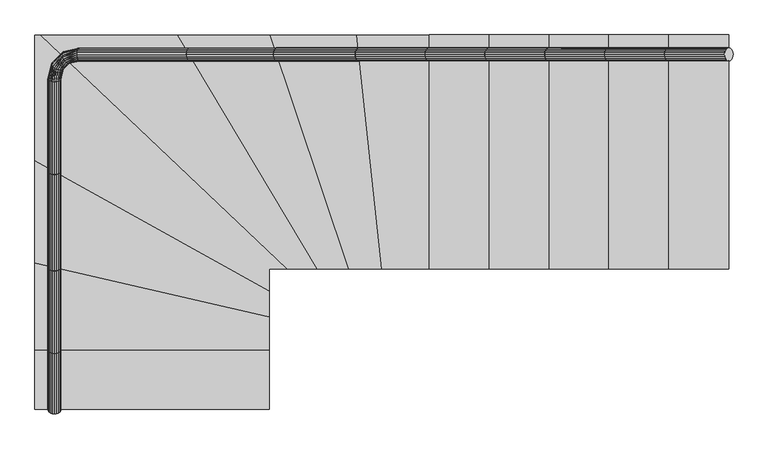
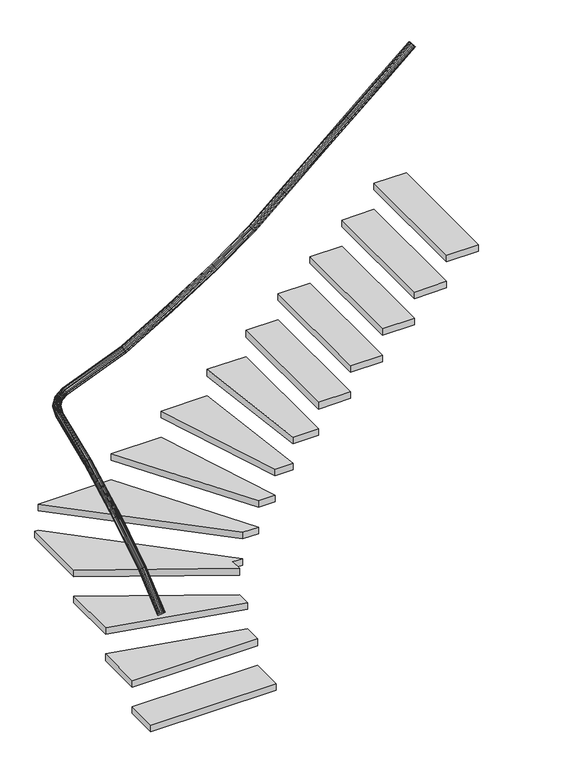
"""IFC4 building model written with IfcOpenShell, lengths in millimetres: stair geometry, 0_3d."""

from ifc_helpers import new_model, si_unit, frame, origin, origin_with_axes, place, context, project, spatial, polyline, outline, extrude, faceted_brep, source, transform, mapped, element, save


def stair_7a128c32(model_context):
    return source(origin(), model_context, "Body", "SolidModel", [
        faceted_brep([(51.2235871, 11.6788974, 875.6088541), (50.0, 16.9018591, 869.5592366), (51.2235871, 22.1248208, 863.5096191), (54.7745751, 26.8365226, 858.0521803), (60.3053687, 30.5757504, 853.7211323), (67.2745751, 32.9764824, 850.9404284), (75.0, 33.8037182, 849.9822631), (82.7254249, 32.9764824, 850.9404284), (89.6946313, 30.5757504, 853.7211323), (95.2254249, 26.8365226, 858.0521803), (98.7764129, 22.1248208, 863.5096191), (100.0, 16.9018591, 869.5592366), (98.7764129, 11.6788974, 875.6088541), (95.2254249, 6.9671956, 881.0662929), (89.6946313, 3.2279679, 885.3973409), (82.7254249, 0.8272359, 888.1780448), (75.0, 0.0, 889.1362101), (67.2745751, 0.8272359, 888.1780448), (60.3053687, 3.2279679, 885.3973409), (54.7745751, 6.9671956, 881.0662929), (51.2235871, 251.6675536, 1061.6862641), (50.0, 246.9018591, 1068.1306652), (51.2235871, 242.1361647, 1074.5750662), (54.7745751, 237.8369696, 1080.3886444), (60.3053687, 234.4251091, 1085.0023262), (67.2745751, 232.2345598, 1087.9644922), (75.0, 231.4797479, 1088.985185), (82.7254249, 232.2345598, 1087.9644922), (89.6946313, 234.4251091, 1085.0023262), (95.2254249, 237.8369696, 1080.3886444), (98.7764129, 242.1361647, 1074.5750662), (100.0, 246.9018591, 1068.1306652), (98.7764129, 251.6675536, 1061.6862641), (95.2254249, 255.9667486, 1055.872686), (89.6946313, 259.3786091, 1051.2590042), (82.7254249, 261.5691584, 1048.2968382), (75.0, 262.3239703, 1047.2761453), (67.2745751, 261.5691584, 1048.2968382), (60.3053687, 259.3786091, 1051.2590042), (54.7745751, 255.9667486, 1055.872686)], [[[0, 1, 2, 3, 4, 5, 6, 7, 8, 9, 10, 11, 12, 13, 14, 15, 16, 17, 18, 19]], [[20, 21, 22, 23, 24, 25, 26, 27, 28, 29, 30, 31, 32, 33, 34, 35, 36, 37, 38, 39]], [[21, 1, 0, 22]], [[22, 0, 19, 23]], [[23, 19, 18, 24]], [[24, 18, 17, 25]], [[25, 17, 16, 26]], [[26, 16, 15, 27]], [[27, 15, 14, 28]], [[28, 14, 13, 29]], [[29, 13, 12, 30]], [[30, 12, 11, 31]], [[31, 11, 10, 32]], [[32, 10, 9, 33]], [[33, 9, 8, 34]], [[34, 8, 7, 35]], [[35, 7, 6, 36]], [[36, 6, 5, 37]], [[37, 5, 4, 38]], [[38, 4, 3, 39]], [[39, 3, 2, 20]], [[20, 2, 1, 21]]]),
        extrude(outline(polyline([(900.0, 373.9346688), (0.0, 579.8690495), (0.0, 973.1970565), (900.0, 473.824936), (900.0, 373.9346688)])), frame((0.0, 0.0, 397.1428571), z_axis=(0.0, 0.0, 1.0), x_axis=(1.0, 0.0, 0.0)), (0.0, 0.0, 1.0), 50.0),
        extrude(outline(polyline([(1.2235871, -7.9923214), (0.0, 0.0), (1.2235871, 7.9923214), (4.7745751, 15.2022986), (10.3053687, 20.924169), (17.2745751, 24.5978359), (25.0, 25.8636953), (32.7254248, 24.5978359), (39.6946313, 20.924169), (45.2254248, 15.2022986), (48.7764129, 7.9923214), (50.0, 0.0), (48.7764129, -7.9923214), (45.2254248, -15.2022987), (39.6946313, -20.9241691), (32.7254248, -24.597836), (25.0, -25.8636953), (17.2745751, -24.597836), (10.3053687, -20.9241691), (4.7745751, -15.2022987), (1.2235871, -7.9923214)])), frame((1744.6018366, 1406.9018591, 2656.7020937), z_axis=(0.7569287102857354, 0.0, 0.6534974579485168), x_axis=(0.0, -1.0, 0.0)), (0.0, 0.0, 1.0), 303.8595272),
        faceted_brep([(1509.6138519, 1405.678272, 2464.383151), (1514.6018366, 1406.9018591, 2458.1306652), (1519.5898213, 1405.678272, 2451.8781793), (1524.0895473, 1402.127284, 2446.2377304), (1527.6605501, 1396.5964904, 2441.7614447), (1529.9532751, 1389.627284, 2438.8874925), (1530.7432942, 1381.9018591, 2437.897196), (1529.9532751, 1374.1764343, 2438.8874925), (1527.6605501, 1367.2072278, 2441.7614447), (1524.0895473, 1361.6764343, 2446.2377304), (1519.5898213, 1358.1254462, 2451.8781793), (1514.6018366, 1356.9018591, 2458.1306652), (1509.6138519, 1358.1254462, 2464.383151), (1505.1141259, 1361.6764343, 2470.0236), (1501.5431231, 1367.2072278, 2474.4998856), (1499.2503981, 1374.1764343, 2477.3738379), (1498.460379, 1381.9018591, 2478.3641344), (1499.2503981, 1389.627284, 2477.3738379), (1501.5431231, 1396.5964904, 2474.4998856), (1505.1141259, 1402.127284, 2470.0236), (1749.8247983, 1405.678272, 2650.6524762), (1744.6018366, 1406.9018591, 2656.7020937), (1739.3788749, 1405.678272, 2662.7517113), (1734.6671731, 1402.127284, 2668.2091501), (1730.9279453, 1396.5964904, 2672.540198), (1728.5272134, 1389.627284, 2675.320902), (1727.6999775, 1381.9018591, 2676.2790673), (1728.5272134, 1374.1764343, 2675.320902), (1730.9279453, 1367.2072278, 2672.540198), (1734.6671731, 1361.6764343, 2668.2091501), (1739.3788749, 1358.1254462, 2662.7517113), (1744.6018366, 1356.9018591, 2656.7020937), (1749.8247983, 1358.1254462, 2650.6524762), (1754.5365001, 1361.6764343, 2645.1950374), (1758.2757279, 1367.2072278, 2640.8639895), (1760.6764598, 1374.1764343, 2638.0832855), (1761.5036957, 1381.9018591, 2637.1251202), (1760.6764598, 1389.627284, 2638.0832855), (1758.2757279, 1396.5964904, 2640.8639895), (1754.5365001, 1402.127284, 2645.1950374)], [[[0, 1, 2, 3, 4, 5, 6, 7, 8, 9, 10, 11, 12, 13, 14, 15, 16, 17, 18, 19]], [[20, 21, 22, 23, 24, 25, 26, 27, 28, 29, 30, 31, 32, 33, 34, 35, 36, 37, 38, 39]], [[21, 1, 0, 22]], [[22, 0, 19, 23]], [[23, 19, 18, 24]], [[24, 18, 17, 25]], [[25, 17, 16, 26]], [[26, 16, 15, 27]], [[27, 15, 14, 28]], [[28, 14, 13, 29]], [[29, 13, 12, 30]], [[30, 12, 11, 31]], [[31, 11, 10, 32]], [[32, 10, 9, 33]], [[33, 9, 8, 34]], [[34, 8, 7, 35]], [[35, 7, 6, 36]], [[36, 6, 5, 37]], [[37, 5, 4, 38]], [[38, 4, 3, 39]], [[39, 3, 2, 20]], [[20, 2, 1, 21]]]),
        faceted_brep([(51.2235871, 242.1361647, 1074.5750662), (50.0, 246.9018591, 1068.1306652), (51.2235871, 251.6675536, 1061.6862641), (54.7745751, 255.9667486, 1055.872686), (60.3053687, 259.3786091, 1051.2590042), (67.2745751, 261.5691584, 1048.2968382), (75.0, 262.3239703, 1047.2761453), (82.7254249, 261.5691584, 1048.2968382), (89.6946313, 259.3786091, 1051.2590042), (95.2254249, 255.9667486, 1055.872686), (98.7764129, 251.6675536, 1061.6862641), (100.0, 246.9018591, 1068.1306652), (98.7764129, 242.1361647, 1074.5750662), (95.2254249, 237.8369696, 1080.3886444), (89.6946313, 234.4251091, 1085.0023262), (82.7254249, 232.2345598, 1087.9644922), (75.0, 231.4797479, 1088.985185), (67.2745751, 232.2345598, 1087.9644922), (60.3053687, 234.4251091, 1085.0023262), (54.7745751, 237.8369696, 1080.3886444), (51.2235871, 566.7337566, 1259.7925307), (50.0, 562.7078511, 1266.7020937), (51.2235871, 558.6819455, 1273.6116568), (54.7745751, 555.0501237, 1279.8448636), (60.3053687, 552.1678935, 1284.7915646), (67.2745751, 550.3173878, 1287.9675421), (75.0, 549.679747, 1289.0619094), (82.7254249, 550.3173878, 1287.9675421), (89.6946313, 552.1678935, 1284.7915646), (95.2254249, 555.0501237, 1279.8448636), (98.7764129, 558.6819455, 1273.6116568), (100.0, 562.7078511, 1266.7020937), (98.7764129, 566.7337566, 1259.7925307), (95.2254249, 570.3655785, 1253.5593239), (89.6946313, 573.2478087, 1248.6126229), (82.7254249, 575.0983143, 1245.4366454), (75.0, 575.7359551, 1244.3422781), (67.2745751, 575.0983143, 1245.4366454), (60.3053687, 573.2478087, 1248.6126229), (54.7745751, 570.3655785, 1253.5593239)], [[[0, 1, 2, 3, 4, 5, 6, 7, 8, 9, 10, 11, 12, 13, 14, 15, 16, 17, 18, 19]], [[20, 21, 22, 23, 24, 25, 26, 27, 28, 29, 30, 31, 32, 33, 34, 35, 36, 37, 38, 39]], [[21, 1, 0, 22]], [[22, 0, 19, 23]], [[23, 19, 18, 24]], [[24, 18, 17, 25]], [[25, 17, 16, 26]], [[26, 16, 15, 27]], [[27, 15, 14, 28]], [[28, 14, 13, 29]], [[29, 13, 12, 30]], [[30, 12, 11, 31]], [[31, 11, 10, 32]], [[32, 10, 9, 33]], [[33, 9, 8, 34]], [[34, 8, 7, 35]], [[35, 7, 6, 36]], [[36, 6, 5, 37]], [[37, 5, 4, 38]], [[38, 4, 3, 39]], [[39, 3, 2, 20]], [[20, 2, 1, 21]]]),
        extrude(outline(polyline([(1.2235871, -7.9923214), (0.0, 0.0), (1.2235871, 7.9923214), (4.7745751, 15.2022986), (10.3053687, 20.9241691), (17.2745751, 24.597836), (25.0, 25.8636953), (32.7254248, 24.597836), (39.6946313, 20.9241691), (45.2254248, 15.2022986), (48.7764129, 7.9923214), (50.0, 0.0), (48.7764129, -7.9923214), (45.2254248, -15.2022986), (39.6946313, -20.924169), (32.7254248, -24.5978359), (25.0, -25.8636953), (17.2745751, -24.5978359), (10.3053687, -20.924169), (4.7745751, -15.2022986), (1.2235871, -7.9923214)])), frame((2434.6018366, 1406.9018591, 3252.4163795), z_axis=(0.7569287102857536, 0.0, 0.6534974579484957), x_axis=(0.0, -1.0, 0.0)), (0.0, 0.0, 1.0), 303.8595272),
        faceted_brep([(925.538539, 1405.678272, 2067.8109967), (929.7020117, 1406.9018591, 2060.987808), (933.8654844, 1405.678272, 2054.1646194), (937.6214074, 1402.127284, 2048.009332), (940.6021247, 1396.5964904, 2043.1244683), (942.515863, 1389.627284, 2039.9881928), (943.1752923, 1381.9018591, 2038.9075058), (942.515863, 1374.1764343, 2039.9881928), (940.6021247, 1367.2072278, 2043.1244683), (937.6214074, 1361.6764343, 2048.009332), (933.8654844, 1358.1254462, 2054.1646194), (929.7020117, 1356.9018591, 2060.987808), (925.538539, 1358.1254462, 2067.8109967), (921.782616, 1361.6764343, 2073.966284), (918.8018987, 1367.2072278, 2078.8511477), (916.8881603, 1374.1764343, 2081.9874233), (916.228731, 1381.9018591, 2083.0681102), (916.8881603, 1389.627284, 2081.9874233), (918.8018987, 1396.5964904, 2078.8511477), (921.782616, 1402.127284, 2073.966284), (1249.3489942, 1405.678272, 2252.9513864), (1244.8437697, 1406.9018591, 2259.5592366), (1240.3385453, 1405.678272, 2266.1670868), (1236.2743236, 1402.127284, 2272.1281145), (1233.048939, 1396.5964904, 2276.858813), (1230.9781146, 1389.627284, 2279.8961083), (1230.2645572, 1381.9018591, 2280.942689), (1230.9781146, 1374.1764343, 2279.8961083), (1233.048939, 1367.2072278, 2276.858813), (1236.2743236, 1361.6764343, 2272.1281145), (1240.3385453, 1358.1254462, 2266.1670868), (1244.8437697, 1356.9018591, 2259.5592366), (1249.3489942, 1358.1254462, 2252.9513864), (1253.4132159, 1361.6764343, 2246.9903587), (1256.6386004, 1367.2072278, 2242.2596602), (1258.7094248, 1374.1764343, 2239.2223649), (1259.4229823, 1381.9018591, 2238.1757842), (1258.7094248, 1389.627284, 2239.2223649), (1256.6386004, 1396.5964904, 2242.2596602), (1253.4132159, 1402.127284, 2246.9903587)], [[[0, 1, 2, 3, 4, 5, 6, 7, 8, 9, 10, 11, 12, 13, 14, 15, 16, 17, 18, 19]], [[20, 21, 22, 23, 24, 25, 26, 27, 28, 29, 30, 31, 32, 33, 34, 35, 36, 37, 38, 39]], [[21, 1, 0, 22]], [[22, 0, 19, 23]], [[23, 19, 18, 24]], [[24, 18, 17, 25]], [[25, 17, 16, 26]], [[26, 16, 15, 27]], [[27, 15, 14, 28]], [[28, 14, 13, 29]], [[29, 13, 12, 30]], [[30, 12, 11, 31]], [[31, 11, 10, 32]], [[32, 10, 9, 33]], [[33, 9, 8, 34]], [[34, 8, 7, 35]], [[35, 7, 6, 36]], [[36, 6, 5, 37]], [[37, 5, 4, 38]], [[38, 4, 3, 39]], [[39, 3, 2, 20]], [[20, 2, 1, 21]]]),
        extrude(outline(polyline([(900.0, 473.824936), (0.0, 973.1970565), (0.0, 1456.9018591), (22.6704161, 1456.9018591), (970.0, 556.9018591), (900.0, 556.9018591), (900.0, 473.824936)])), frame((0.0, 0.0, 595.7142857), z_axis=(0.0, 0.0, 1.0), x_axis=(1.0, 0.0, 0.0)), (0.0, 0.0, 1.0), 50.0),
        faceted_brep([(1240.3385453, 1405.678272, 2266.1670868), (1244.8437697, 1406.9018591, 2259.5592366), (1249.3489942, 1405.678272, 2252.9513864), (1253.4132159, 1402.127284, 2246.9903587), (1256.6386004, 1396.5964904, 2242.2596602), (1258.7094248, 1389.627284, 2239.2223649), (1259.4229823, 1381.9018591, 2238.1757842), (1258.7094248, 1374.1764343, 2239.2223649), (1256.6386004, 1367.2072278, 2242.2596602), (1253.4132159, 1361.6764343, 2246.9903587), (1249.3489942, 1358.1254462, 2252.9513864), (1244.8437697, 1356.9018591, 2259.5592366), (1240.3385453, 1358.1254462, 2266.1670868), (1236.2743236, 1361.6764343, 2272.1281145), (1233.048939, 1367.2072278, 2276.858813), (1230.9781146, 1374.1764343, 2279.8961083), (1230.2645572, 1381.9018591, 2280.942689), (1230.9781146, 1389.627284, 2279.8961083), (1233.048939, 1396.5964904, 2276.858813), (1236.2743236, 1402.127284, 2272.1281145), (1519.5898213, 1405.678272, 2451.8781793), (1514.6018366, 1406.9018591, 2458.1306652), (1509.6138519, 1405.678272, 2464.383151), (1505.1141259, 1402.127284, 2470.0236), (1501.5431231, 1396.5964904, 2474.4998856), (1499.2503981, 1389.627284, 2477.3738379), (1498.460379, 1381.9018591, 2478.3641344), (1499.2503981, 1374.1764343, 2477.3738379), (1501.5431231, 1367.2072278, 2474.4998856), (1505.1141259, 1361.6764343, 2470.0236), (1509.6138519, 1358.1254462, 2464.383151), (1514.6018366, 1356.9018591, 2458.1306652), (1519.5898213, 1358.1254462, 2451.8781793), (1524.0895473, 1361.6764343, 2446.2377304), (1527.6605501, 1367.2072278, 2441.7614447), (1529.9532751, 1374.1764343, 2438.8874925), (1530.7432942, 1381.9018591, 2437.897196), (1529.9532751, 1389.627284, 2438.8874925), (1527.6605501, 1396.5964904, 2441.7614447), (1524.0895473, 1402.127284, 2446.2377304)], [[[0, 1, 2, 3, 4, 5, 6, 7, 8, 9, 10, 11, 12, 13, 14, 15, 16, 17, 18, 19]], [[20, 21, 22, 23, 24, 25, 26, 27, 28, 29, 30, 31, 32, 33, 34, 35, 36, 37, 38, 39]], [[21, 1, 0, 22]], [[22, 0, 19, 23]], [[23, 19, 18, 24]], [[24, 18, 17, 25]], [[25, 17, 16, 26]], [[26, 16, 15, 27]], [[27, 15, 14, 28]], [[28, 14, 13, 29]], [[29, 13, 12, 30]], [[30, 12, 11, 31]], [[31, 11, 10, 32]], [[32, 10, 9, 33]], [[33, 9, 8, 34]], [[34, 8, 7, 35]], [[35, 7, 6, 36]], [[36, 6, 5, 37]], [[37, 5, 4, 38]], [[38, 4, 3, 39]], [[39, 3, 2, 20]], [[20, 2, 1, 21]]]),
        extrude(outline(polyline([(1204.4816265, 556.9018591), (904.7220467, 1456.9018591), (1236.8921564, 1456.9018591), (1332.3115168, 556.9018591), (1204.4816265, 556.9018591)])), frame((0.0, 0.0, 1191.4285714), z_axis=(0.0, 0.0, 1.0), x_axis=(1.0, 0.0, 0.0)), (0.0, 0.0, 1.0), 50.0),
        extrude(outline(polyline([(900.0, 16.9018591), (0.0, 16.9018591), (0.0, 246.9018591), (900.0, 246.9018591), (900.0, 16.9018591)])), origin_with_axes(), (0.0, 0.0, 1.0), 50.0),
        faceted_brep([(589.9532071, 1405.678272, 1869.6030507), (593.5012683, 1406.9018591, 1862.4163795), (597.0493296, 1405.678272, 1855.2297082), (600.2500819, 1402.127284, 1848.7465184), (602.7902133, 1396.5964904, 1843.6014299), (604.421078, 1389.627284, 1840.2980797), (604.9830357, 1381.9018591, 1839.1598228), (604.421078, 1374.1764343, 1840.2980797), (602.7902133, 1367.2072278, 1843.6014299), (600.2500819, 1361.6764343, 1848.7465184), (597.0493296, 1358.1254462, 1855.2297082), (593.5012683, 1356.9018591, 1862.4163795), (589.9532071, 1358.1254462, 1869.6030507), (586.7524548, 1361.6764343, 1876.0862405), (584.2123234, 1367.2072278, 1881.231329), (582.5814586, 1374.1764343, 1884.5346792), (582.019501, 1381.9018591, 1885.6729361), (582.5814586, 1389.627284, 1884.5346792), (584.2123234, 1396.5964904, 1881.231329), (586.7524548, 1402.127284, 1876.0862405), (933.8654844, 1405.678272, 2054.1646194), (929.7020117, 1406.9018591, 2060.987808), (925.538539, 1405.678272, 2067.8109967), (921.782616, 1402.127284, 2073.966284), (918.8018987, 1396.5964904, 2078.8511477), (916.8881603, 1389.627284, 2081.9874233), (916.228731, 1381.9018591, 2083.0681102), (916.8881603, 1374.1764343, 2081.9874233), (918.8018987, 1367.2072278, 2078.8511477), (921.782616, 1361.6764343, 2073.966284), (925.538539, 1358.1254462, 2067.8109967), (929.7020117, 1356.9018591, 2060.987808), (933.8654844, 1358.1254462, 2054.1646194), (937.6214074, 1361.6764343, 2048.009332), (940.6021247, 1367.2072278, 2043.1244683), (942.515863, 1374.1764343, 2039.9881928), (943.1752923, 1381.9018591, 2038.9075058), (942.515863, 1389.627284, 2039.9881928), (940.6021247, 1396.5964904, 2043.1244683), (937.6214074, 1402.127284, 2048.009332)], [[[0, 1, 2, 3, 4, 5, 6, 7, 8, 9, 10, 11, 12, 13, 14, 15, 16, 17, 18, 19]], [[20, 21, 22, 23, 24, 25, 26, 27, 28, 29, 30, 31, 32, 33, 34, 35, 36, 37, 38, 39]], [[21, 1, 0, 22]], [[22, 0, 19, 23]], [[23, 19, 18, 24]], [[24, 18, 17, 25]], [[25, 17, 16, 26]], [[26, 16, 15, 27]], [[27, 15, 14, 28]], [[28, 14, 13, 29]], [[29, 13, 12, 30]], [[30, 12, 11, 31]], [[31, 11, 10, 32]], [[32, 10, 9, 33]], [[33, 9, 8, 34]], [[34, 8, 7, 35]], [[35, 7, 6, 36]], [[36, 6, 5, 37]], [[37, 5, 4, 38]], [[38, 4, 3, 39]], [[39, 3, 2, 20]], [[20, 2, 1, 21]]]),
        extrude(outline(polyline([(1332.3115168, 556.9018591), (1236.8921564, 1456.9018591), (1514.6018366, 1456.9018591), (1514.6018366, 556.9018591), (1332.3115168, 556.9018591)])), frame((0.0, 0.0, 1390.0), z_axis=(0.0, 0.0, 1.0), x_axis=(1.0, 0.0, 0.0)), (0.0, 0.0, 1.0), 50.0),
        extrude(outline(polyline([(1744.6018366, 556.9018591), (1744.6018366, 1456.9018591), (1974.6018366, 1456.9018591), (1974.6018366, 556.9018591), (1744.6018366, 556.9018591)])), frame((0.0, 0.0, 1787.1428571), z_axis=(0.0, 0.0, 1.0), x_axis=(1.0, 0.0, 0.0)), (0.0, 0.0, 1.0), 50.0),
        extrude(outline(polyline([(1974.6018366, 556.9018591), (1974.6018366, 1456.9018591), (2204.6018366, 1456.9018591), (2204.6018366, 556.9018591), (1974.6018366, 556.9018591)])), frame((0.0, 0.0, 1985.7142857), z_axis=(0.0, 0.0, 1.0), x_axis=(1.0, 0.0, 0.0)), (0.0, 0.0, 1.0), 50.0),
        faceted_brep([(51.2235871, 1283.3224302, 1620.3777918), (50.0, 1286.3944101, 1612.9994356), (51.2235871, 1289.46639, 1605.6210794), (54.7745751, 1292.2376632, 1598.9649681), (60.3053687, 1294.436958, 1593.6826483), (67.2745751, 1295.8489921, 1590.2911902), (75.0, 1296.335546, 1589.1225734), (82.7254249, 1295.8489921, 1590.2911902), (89.6946313, 1294.436958, 1593.6826483), (95.2254249, 1292.2376632, 1598.9649681), (98.7764129, 1289.46639, 1605.6210794), (100.0, 1286.3944101, 1612.9994356), (98.7764129, 1283.3224302, 1620.3777918), (95.2254249, 1280.5511571, 1627.0339031), (89.6946313, 1278.3518623, 1632.3162229), (82.7254249, 1276.9398281, 1635.707681), (75.0, 1276.4532743, 1636.8762979), (67.2745751, 1276.9398281, 1635.707681), (60.3053687, 1278.3518623, 1632.3162229), (54.7745751, 1280.5511571, 1627.0339031), (65.0056921, 1348.8501513, 1638.9123688), (64.1990579, 1344.8271855, 1645.879395), (65.6181519, 1340.0232633, 1652.1644401), (69.1240635, 1334.9086261, 1657.1522801), (74.3736094, 1329.9839302, 1660.3546705), (80.8529277, 1325.7312391, 1661.4581391), (87.9277774, 1322.5668359, 1660.3546705), (94.9056231, 1320.8004745, 1657.1522801), (101.1034244, 1320.6050585, 1652.1644401), (105.9144976, 1321.9997167, 1645.879395), (108.8679012, 1324.8479302, 1638.9123688), (109.6745354, 1328.870896, 1631.9453426), (108.2554414, 1333.6748181, 1625.6602975), (104.7495298, 1338.7894554, 1620.6724574), (99.4999839, 1343.7141513, 1617.470067), (93.0206656, 1347.9668423, 1616.3665985), (85.9458159, 1351.1312455, 1617.470067), (78.9679702, 1352.8976069, 1620.6724574), (72.7701688, 1353.0930229, 1625.6602975), (67.9590957, 1351.6983647, 1631.9453426), (108.2142101, 1391.9456089, 1666.2859781), (105.3846216, 1389.0124344, 1673.2691208), (104.0019016, 1384.2169558, 1679.5687049), (104.2014005, 1378.028588, 1684.5680831), (105.96359, 1371.0530916, 1687.7778814), (109.1159746, 1363.9732768, 1688.8839026), (113.3499769, 1357.4821652, 1687.7778814), (118.2511434, 1352.215152, 1684.5680831), (123.3397137, 1348.6878091, 1679.5687049), (128.1175831, 1347.2454175, 1673.2691208), (132.1170605, 1348.0291684, 1666.2859781), (134.946649, 1350.962343, 1659.3028354), (136.329369, 1355.7578216, 1653.0032514), (136.1298701, 1361.9461894, 1648.0038732), (134.3676806, 1368.9216857, 1644.7940748), (131.215296, 1376.0015006, 1643.6880537), (126.9812936, 1382.4926122, 1644.7940748), (122.0801271, 1387.7596254, 1648.0038732), (116.9915569, 1391.2869683, 1653.0032514), (112.2136875, 1392.7293599, 1659.3028354), (170.8141891, 1406.9018591, 1691.7803901), (167.8223333, 1405.678272, 1699.1915978), (165.1233413, 1402.127284, 1705.8773449), (162.981409, 1396.5964904, 1711.1831838), (161.6062039, 1389.627284, 1714.5897421), (161.1323405, 1381.9018591, 1715.7635621), (161.6062039, 1374.1764343, 1714.5897421), (162.981409, 1367.2072278, 1711.1831838), (165.1233413, 1361.6764343, 1705.8773449), (167.8223333, 1358.1254462, 1699.1915978), (170.8141891, 1356.9018591, 1691.7803901), (173.8060448, 1358.1254462, 1684.3691823), (176.5050369, 1361.6764343, 1677.6834352), (178.6469691, 1367.2072278, 1672.3775963), (180.0221742, 1374.1764343, 1668.971038), (180.4960376, 1381.9018591, 1667.797218), (180.0221742, 1389.627284, 1668.971038), (178.6469691, 1396.5964904, 1672.3775963), (176.5050369, 1402.127284, 1677.6834352), (173.8060448, 1405.678272, 1684.3691823), (597.0493296, 1405.678272, 1855.2297082), (593.5012683, 1406.9018591, 1862.4163795), (589.9532071, 1405.678272, 1869.6030507), (586.7524548, 1402.127284, 1876.0862405), (584.2123234, 1396.5964904, 1881.231329), (582.5814586, 1389.627284, 1884.5346792), (582.019501, 1381.9018591, 1885.6729361), (582.5814586, 1374.1764343, 1884.5346792), (584.2123234, 1367.2072278, 1881.231329), (586.7524548, 1361.6764343, 1876.0862405), (589.9532071, 1358.1254462, 1869.6030507), (593.5012683, 1356.9018591, 1862.4163795), (597.0493296, 1358.1254462, 1855.2297082), (600.2500819, 1361.6764343, 1848.7465184), (602.7902133, 1367.2072278, 1843.6014299), (604.421078, 1374.1764343, 1840.2980797), (604.9830357, 1381.9018591, 1839.1598228), (604.421078, 1389.627284, 1840.2980797), (602.7902133, 1396.5964904, 1843.6014299), (600.2500819, 1402.127284, 1848.7465184)], [[[0, 1, 2, 3, 4, 5, 6, 7, 8, 9, 10, 11, 12, 13, 14, 15, 16, 17, 18, 19]], [[20, 1, 0]], [[20, 0, 21]], [[21, 0, 19]], [[21, 19, 22]], [[22, 19, 18]], [[22, 18, 23]], [[23, 18, 17]], [[23, 17, 24]], [[24, 17, 16]], [[24, 16, 25]], [[25, 16, 15]], [[25, 15, 26]], [[26, 15, 14]], [[26, 14, 27]], [[27, 14, 13]], [[27, 13, 28]], [[28, 13, 12]], [[28, 12, 29]], [[29, 12, 11]], [[29, 11, 30]], [[30, 11, 10]], [[30, 10, 31]], [[31, 10, 9]], [[31, 9, 32]], [[32, 9, 8]], [[32, 8, 33]], [[33, 8, 7]], [[33, 7, 34]], [[34, 7, 6]], [[34, 6, 35]], [[35, 6, 5]], [[35, 5, 36]], [[36, 5, 4]], [[36, 4, 37]], [[37, 4, 3]], [[37, 3, 38]], [[38, 3, 2]], [[38, 2, 39]], [[39, 2, 1]], [[39, 1, 20]], [[40, 20, 21]], [[40, 21, 41]], [[41, 21, 22]], [[41, 22, 42]], [[42, 22, 23]], [[42, 23, 43]], [[43, 23, 24]], [[43, 24, 44]], [[44, 24, 25]], [[44, 25, 45]], [[45, 25, 26]], [[45, 26, 46]], [[46, 26, 27]], [[46, 27, 47]], [[47, 27, 28]], [[47, 28, 48]], [[48, 28, 29]], [[48, 29, 49]], [[49, 29, 30]], [[49, 30, 50]], [[50, 30, 31]], [[50, 31, 51]], [[51, 31, 32]], [[51, 32, 52]], [[52, 32, 33]], [[52, 33, 53]], [[53, 33, 34]], [[53, 34, 54]], [[54, 34, 35]], [[54, 35, 55]], [[55, 35, 36]], [[55, 36, 56]], [[56, 36, 37]], [[56, 37, 57]], [[57, 37, 38]], [[57, 38, 58]], [[58, 38, 39]], [[58, 39, 59]], [[59, 39, 20]], [[59, 20, 40]], [[60, 40, 41]], [[60, 41, 61]], [[61, 41, 42]], [[61, 42, 62]], [[62, 42, 43]], [[62, 43, 63]], [[63, 43, 44]], [[63, 44, 64]], [[64, 44, 45]], [[64, 45, 65]], [[65, 45, 46]], [[65, 46, 66]], [[66, 46, 47]], [[66, 47, 67]], [[67, 47, 48]], [[67, 48, 68]], [[68, 48, 49]], [[68, 49, 69]], [[69, 49, 50]], [[69, 50, 70]], [[70, 50, 51]], [[70, 51, 71]], [[71, 51, 52]], [[71, 52, 72]], [[72, 52, 53]], [[72, 53, 73]], [[73, 53, 54]], [[73, 54, 74]], [[74, 54, 55]], [[74, 55, 75]], [[75, 55, 56]], [[75, 56, 76]], [[76, 56, 57]], [[76, 57, 77]], [[77, 57, 58]], [[77, 58, 78]], [[78, 58, 59]], [[78, 59, 79]], [[79, 59, 40]], [[79, 40, 60]], [[80, 81, 82, 83, 84, 85, 86, 87, 88, 89, 90, 91, 92, 93, 94, 95, 96, 97, 98, 99]], [[81, 60, 61, 82]], [[82, 61, 62, 83]], [[83, 62, 63, 84]], [[84, 63, 64, 85]], [[85, 64, 65, 86]], [[86, 65, 66, 87]], [[87, 66, 67, 88]], [[88, 67, 68, 89]], [[89, 68, 69, 90]], [[90, 69, 70, 91]], [[91, 70, 71, 92]], [[92, 71, 72, 93]], [[93, 72, 73, 94]], [[94, 73, 74, 95]], [[95, 74, 75, 96]], [[96, 75, 76, 97]], [[97, 76, 77, 98]], [[98, 77, 78, 99]], [[99, 78, 79, 80]], [[80, 79, 60, 81]]]),
        faceted_brep([(51.2235871, 558.6819455, 1273.6116568), (50.0, 562.7078511, 1266.7020937), (51.2235871, 566.7337566, 1259.7925307), (54.7745751, 570.3655785, 1253.5593239), (60.3053687, 573.2478087, 1248.6126229), (67.2745751, 575.0983143, 1245.4366454), (75.0, 575.7359551, 1244.3422781), (82.7254249, 575.0983143, 1245.4366454), (89.6946313, 573.2478087, 1248.6126229), (95.2254249, 570.3655785, 1253.5593239), (98.7764129, 566.7337566, 1259.7925307), (100.0, 562.7078511, 1266.7020937), (98.7764129, 558.6819455, 1273.6116568), (95.2254249, 555.0501237, 1279.8448636), (89.6946313, 552.1678935, 1284.7915646), (82.7254249, 550.3173878, 1287.9675421), (75.0, 549.679747, 1289.0619094), (67.2745751, 550.3173878, 1287.9675421), (60.3053687, 552.1678935, 1284.7915646), (54.7745751, 555.0501237, 1279.8448636), (51.2235871, 935.0213576, 1458.0478269), (50.0, 931.5827131, 1465.2735223), (51.2235871, 928.1440687, 1472.4992177), (54.7745751, 925.0420228, 1479.0176117), (60.3053687, 922.5802252, 1484.1906384), (67.2745751, 920.9996538, 1487.511926), (75.0, 920.4550261, 1488.6563638), (82.7254249, 920.9996538, 1487.511926), (89.6946313, 922.5802252, 1484.1906384), (95.2254249, 925.0420228, 1479.0176117), (98.7764129, 928.1440687, 1472.4992177), (100.0, 931.5827131, 1465.2735223), (98.7764129, 935.0213576, 1458.0478269), (95.2254249, 938.1234035, 1451.529433), (89.6946313, 940.5852011, 1446.3564062), (82.7254249, 942.1657724, 1443.0351186), (75.0, 942.7104002, 1441.8906809), (67.2745751, 942.1657724, 1443.0351186), (60.3053687, 940.5852011, 1446.3564062), (54.7745751, 938.1234035, 1451.529433)], [[[0, 1, 2, 3, 4, 5, 6, 7, 8, 9, 10, 11, 12, 13, 14, 15, 16, 17, 18, 19]], [[20, 21, 22, 23, 24, 25, 26, 27, 28, 29, 30, 31, 32, 33, 34, 35, 36, 37, 38, 39]], [[21, 1, 0, 22]], [[22, 0, 19, 23]], [[23, 19, 18, 24]], [[24, 18, 17, 25]], [[25, 17, 16, 26]], [[26, 16, 15, 27]], [[27, 15, 14, 28]], [[28, 14, 13, 29]], [[29, 13, 12, 30]], [[30, 12, 11, 31]], [[31, 11, 10, 32]], [[32, 10, 9, 33]], [[33, 9, 8, 34]], [[34, 8, 7, 35]], [[35, 7, 6, 36]], [[36, 6, 5, 37]], [[37, 5, 4, 38]], [[38, 4, 3, 39]], [[39, 3, 2, 20]], [[20, 2, 1, 21]]]),
        extrude(outline(polyline([(1514.6018366, 556.9018591), (1514.6018366, 1456.9018591), (1744.6018366, 1456.9018591), (1744.6018366, 556.9018591), (1514.6018366, 556.9018591)])), frame((0.0, 0.0, 1588.5714286), z_axis=(0.0, 0.0, 1.0), x_axis=(1.0, 0.0, 0.0)), (0.0, 0.0, 1.0), 50.0),
        extrude(outline(polyline([(970.0, 556.9018591), (22.6704161, 1456.9018591), (548.8803485, 1456.9018591), (1084.3313864, 556.9018591), (970.0, 556.9018591)])), frame((0.0, 0.0, 794.2857143), z_axis=(0.0, 0.0, 1.0), x_axis=(1.0, 0.0, 0.0)), (0.0, 0.0, 1.0), 50.0),
        extrude(outline(polyline([(2204.6018366, 556.9018591), (2204.6018366, 1456.9018591), (2434.6018366, 1456.9018591), (2434.6018366, 556.9018591), (2204.6018366, 556.9018591)])), frame((0.0, 0.0, 2184.2857143), z_axis=(0.0, 0.0, 1.0), x_axis=(1.0, 0.0, 0.0)), (0.0, 0.0, 1.0), 50.0),
        faceted_brep([(51.2235871, 928.1440687, 1472.4992177), (50.0, 931.5827131, 1465.2735223), (51.2235871, 935.0213576, 1458.0478269), (54.7745751, 938.1234035, 1451.529433), (60.3053687, 940.5852011, 1446.3564062), (67.2745751, 942.1657724, 1443.0351186), (75.0, 942.7104002, 1441.8906809), (82.7254249, 942.1657724, 1443.0351186), (89.6946313, 940.5852011, 1446.3564062), (95.2254249, 938.1234035, 1451.529433), (98.7764129, 935.0213576, 1458.0478269), (100.0, 931.5827131, 1465.2735223), (98.7764129, 928.1440687, 1472.4992177), (95.2254249, 925.0420228, 1479.0176117), (89.6946313, 922.5802252, 1484.1906384), (82.7254249, 920.9996538, 1487.511926), (75.0, 920.4550261, 1488.6563638), (67.2745751, 920.9996538, 1487.511926), (60.3053687, 922.5802252, 1484.1906384), (54.7745751, 925.0420228, 1479.0176117), (51.2235871, 1289.46639, 1605.6210794), (50.0, 1286.3944101, 1612.9994356), (51.2235871, 1283.3224302, 1620.3777918), (54.7745751, 1280.5511571, 1627.0339031), (60.3053687, 1278.3518623, 1632.3162229), (67.2745751, 1276.9398281, 1635.707681), (75.0, 1276.4532743, 1636.8762979), (82.7254249, 1276.9398281, 1635.707681), (89.6946313, 1278.3518623, 1632.3162229), (95.2254249, 1280.5511571, 1627.0339031), (98.7764129, 1283.3224302, 1620.3777918), (100.0, 1286.3944101, 1612.9994356), (98.7764129, 1289.46639, 1605.6210794), (95.2254249, 1292.2376632, 1598.9649681), (89.6946313, 1294.436958, 1593.6826483), (82.7254249, 1295.8489921, 1590.2911902), (75.0, 1296.335546, 1589.1225734), (67.2745751, 1295.8489921, 1590.2911902), (60.3053687, 1294.436958, 1593.6826483), (54.7745751, 1292.2376632, 1598.9649681)], [[[0, 1, 2, 3, 4, 5, 6, 7, 8, 9, 10, 11, 12, 13, 14, 15, 16, 17, 18, 19]], [[20, 21, 22, 23, 24, 25, 26, 27, 28, 29, 30, 31, 32, 33, 34, 35, 36, 37, 38, 39]], [[21, 1, 0, 22]], [[22, 0, 19, 23]], [[23, 19, 18, 24]], [[24, 18, 17, 25]], [[25, 17, 16, 26]], [[26, 16, 15, 27]], [[27, 15, 14, 28]], [[28, 14, 13, 29]], [[29, 13, 12, 30]], [[30, 12, 11, 31]], [[31, 11, 10, 32]], [[32, 10, 9, 33]], [[33, 9, 8, 34]], [[34, 8, 7, 35]], [[35, 7, 6, 36]], [[36, 6, 5, 37]], [[37, 5, 4, 38]], [[38, 4, 3, 39]], [[39, 3, 2, 20]], [[20, 2, 1, 21]]]),
        extrude(outline(polyline([(2434.6018366, 556.9018591), (2434.6018366, 1456.9018591), (2664.6018366, 1456.9018591), (2664.6018366, 556.9018591), (2434.6018366, 556.9018591)])), frame((0.0, 0.0, 2382.8571429), z_axis=(0.0, 0.0, 1.0), x_axis=(1.0, 0.0, 0.0)), (0.0, 0.0, 1.0), 50.0),
        extrude(outline(polyline([(1084.3313864, 556.9018591), (548.8803485, 1456.9018591), (904.7220467, 1456.9018591), (1204.4816265, 556.9018591), (1084.3313864, 556.9018591)])), frame((0.0, 0.0, 992.8571429), z_axis=(0.0, 0.0, 1.0), x_axis=(1.0, 0.0, 0.0)), (0.0, 0.0, 1.0), 50.0),
        extrude(outline(polyline([(900.0, 246.9018591), (0.0, 246.9018591), (0.0, 579.8690495), (900.0, 373.9346688), (900.0, 246.9018591)])), frame((0.0, 0.0, 198.5714286), z_axis=(0.0, 0.0, 1.0), x_axis=(1.0, 0.0, 0.0)), (0.0, 0.0, 1.0), 50.0),
        extrude(outline(polyline([(1.2235871, -7.9923214), (0.0, 0.0), (1.2235871, 7.9923214), (4.7745751, 15.2022986), (10.3053687, 20.9241691), (17.2745751, 24.5978359), (25.0, 25.8636953), (32.7254248, 24.5978359), (39.6946313, 20.9241691), (45.2254248, 15.2022986), (48.7764129, 7.9923214), (50.0, 0.0), (48.7764129, -7.9923214), (45.2254248, -15.2022986), (39.6946313, -20.9241691), (32.7254248, -24.5978359), (25.0, -25.8636953), (17.2745751, -24.5978359), (10.3053687, -20.9241691), (4.7745751, -15.2022986), (1.2235871, -7.9923214)])), frame((2204.6018366, 1406.9018591, 3053.8449509), z_axis=(0.7569287102857968, 0.0, 0.6534974579484456), x_axis=(0.0, -1.0, 0.0)), (0.0, 0.0, 1.0), 303.8595272),
        extrude(outline(polyline([(1.2235871, -7.9923214), (0.0, 0.0), (1.2235871, 7.9923214), (4.7745751, 15.2022986), (10.3053687, 20.924169), (17.2745751, 24.5978359), (25.0, 25.8636953), (32.7254248, 24.5978359), (39.6946313, 20.924169), (45.2254248, 15.2022986), (48.7764129, 7.9923214), (50.0, 0.0), (48.7764129, -7.9923214), (45.2254248, -15.2022986), (39.6946313, -20.9241691), (32.7254248, -24.5978359), (25.0, -25.8636953), (17.2745751, -24.5978359), (10.3053687, -20.9241691), (4.7745751, -15.2022986), (1.2235871, -7.9923214)])), frame((1974.6018366, 1406.9018591, 2855.2735223), z_axis=(0.7569287102857382, 0.0, 0.6534974579485135), x_axis=(0.0, -1.0, 0.0)), (0.0, 0.0, 1.0), 303.8595272),
    ])


if __name__ == "__main__":
    model = new_model("IFC4")
    model_context = context("Model", 3, world=origin())
    ifc_project = project(units=[si_unit("LENGTHUNIT", "METRE", prefix="MILLI")], contexts=[model_context])
    site = spatial("IfcSite", under=ifc_project)
    building = spatial("IfcBuilding", under=site)
    placement = place(None, origin())
    stair_shape = stair_7a128c32(model_context)
    element("IfcStair", 1, ObjectType="0_3d", at=placement, inside=building, context=model_context, shape_type="MappedRepresentation", body=[
        mapped(stair_shape, transform((0.0, 0.0, 0.0), x_axis=(1.0, 0.0, 0.0), y_axis=(0.0, 1.0, 0.0), z_axis=(0.0, 0.0, 1.0))),
    ])
    save(model, "model.ifc")

# Revit data of these elements
# Element 1 (IfcStair, "0_3d")
#   Materials on its faces: "*1", "weiss"
# Materials
#   "*1": class "Unassigned", colour RGB 175 175 175, transparency 0
#   "weiss": class "Unassigned", colour RGB 255 255 255, transparency 0
